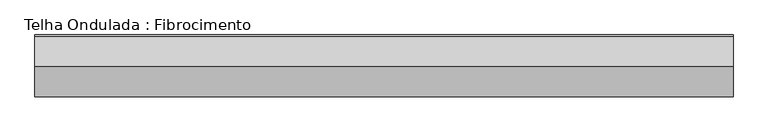
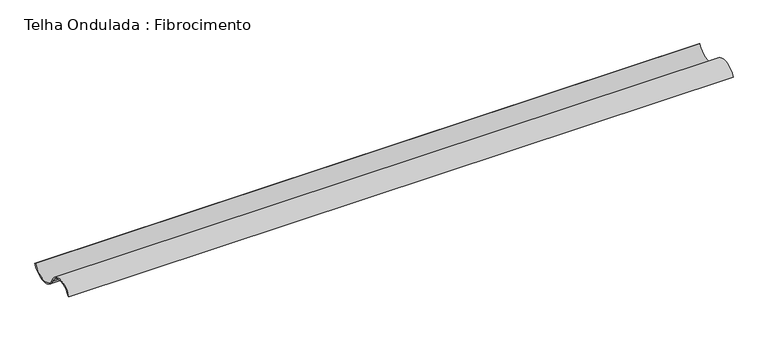
"""IFC4 building model written with IfcOpenShell, lengths in millimetres: beam geometry, Telha Ondulada : Fibrocimento."""

import ifcopenshell
import ifcopenshell.guid

model = None  # the IFC model being written
_history = None  # IfcOwnerHistory: only IFC2X3 demands one
_inside = {}  # id of a spatial element -> (the spatial element, [elements in it])
_under = {}  # id of a project, library or spatial element -> (it, [spatial elements below it])
_declared = {}  # id of a project -> (the project, [libraries it declares])
_typed = {}  # id of a type object -> (the type object, [elements of that type])
_made_of = {}  # id of a material, layer set ... -> (it, [elements and type objects made of it])


def new_model(schema):
    """Start an empty IFC model of exactly this schema.

    Asked for "IFC4X3", IfcOpenShell would pick the latest addendum, in which some entities
    have other attributes; the version numbers below select the first issue.
    IFC2X3 requires an IfcOwnerHistory on every rooted entity: one is made here for all.
    """
    global model, _history
    if schema == "IFC4X3":
        model = ifcopenshell.file(schema_version=(4, 3, 0, 0))
    else:
        model = ifcopenshell.file(schema=schema)
    _inside.clear()
    _under.clear()
    _declared.clear()
    _typed.clear()
    _made_of.clear()
    _history = None
    if model.schema == "IFC2X3":
        org = make("IfcOrganization", Name="unknown")
        user = make(
            "IfcPersonAndOrganization",
            ThePerson=make("IfcPerson", FamilyName="unknown"),
            TheOrganization=org,
        )
        app = make(
            "IfcApplication",
            ApplicationDeveloper=org,
            Version="unknown",
            ApplicationFullName="unknown",
            ApplicationIdentifier="unknown",
        )
        _history = make(
            "IfcOwnerHistory",
            OwningUser=user,
            OwningApplication=app,
            ChangeAction="ADDED",
            CreationDate=0,
        )
    return model


def make(cls, **values):
    """One entity of the class cls with the attributes given. An attribute that is None is left unset."""
    return model.create_entity(
        cls, **{name: value for name, value in values.items() if value is not None}
    )


def rooted(cls, **values):
    """An entity with a GlobalId (a new one), such as an element, a storey or a relation."""
    return make(cls, GlobalId=ifcopenshell.guid.new(), OwnerHistory=_history, **values)


def si_unit(unit_type, name, prefix=None):
    """IfcSIUnit, for example si_unit("LENGTHUNIT", "METRE", prefix="MILLI")."""
    return make("IfcSIUnit", UnitType=unit_type, Prefix=prefix, Name=name)


def assignment(units):
    """IfcUnitAssignment: the units of a project."""
    return None if units is None else make("IfcUnitAssignment", Units=units)


def point(xyz):
    """IfcCartesianPoint."""
    return None if xyz is None else make("IfcCartesianPoint", Coordinates=xyz)


def direction(xyz):
    """IfcDirection."""
    return None if xyz is None else make("IfcDirection", DirectionRatios=xyz)


def frame(location, z_axis=None, x_axis=None):
    """IfcAxis2Placement3D, a coordinate frame: its origin and axes. An axis left out is left unset."""
    return make(
        "IfcAxis2Placement3D",
        Location=point(location),
        Axis=direction(z_axis),
        RefDirection=direction(x_axis),
    )


def frame_2d(location, x_axis=None):
    """IfcAxis2Placement2D, a coordinate frame in the plane: its origin and x axis."""
    return make(
        "IfcAxis2Placement2D", Location=point(location), RefDirection=direction(x_axis)
    )


def origin():
    """The frame at (0, 0, 0) with its axes left unset."""
    return frame((0.0, 0.0, 0.0))


def place(relative_to, where):
    """IfcLocalPlacement: puts the frame where relative to a parent placement (None: the world)."""
    return make(
        "IfcLocalPlacement", PlacementRelTo=relative_to, RelativePlacement=where
    )


def context(
    kind, dimensions, precision=None, world=None, true_north=None, identifier=None
):
    """IfcGeometricRepresentationContext, for example the 3D "Model" context."""
    return make(
        "IfcGeometricRepresentationContext",
        ContextIdentifier=identifier,
        ContextType=kind,
        CoordinateSpaceDimension=dimensions,
        Precision=precision,
        WorldCoordinateSystem=world,
        TrueNorth=true_north,
    )


def project(units=None, contexts=None):
    """IfcProject with its units and contexts."""
    return rooted(
        "IfcProject",
        Name="project",
        RepresentationContexts=contexts,
        UnitsInContext=assignment(units),
    )


def spatial(cls, under=None, at=None, **own):
    """A site, building, storey or space (cls), placed at a placement, below another one or the project."""
    s = rooted(cls, ObjectPlacement=at, **own)
    if under is not None:
        _under.setdefault(under.id(), (under, []))[1].append(s)
    return s


def polyline(points):
    """IfcPolyline through the points."""
    return make("IfcPolyline", Points=[point(p) for p in points])


def circle_curve(where, radius):
    """IfcCircle in the frame where."""
    return make("IfcCircle", Position=where, Radius=radius)


def trimmed(basis, trim1, trim2, sense, master):
    """IfcTrimmedCurve: the piece of a basis curve between two trims."""
    return make(
        "IfcTrimmedCurve",
        BasisCurve=basis,
        Trim1=trim1,
        Trim2=trim2,
        SenseAgreement=sense,
        MasterRepresentation=master,
    )


def segment(curve, same_sense, transition):
    """IfcCompositeCurveSegment."""
    return make(
        "IfcCompositeCurveSegment",
        Transition=transition,
        SameSense=same_sense,
        ParentCurve=curve,
    )


def composite_curve(segments, self_intersect=None):
    """IfcCompositeCurve: segments joined end to end."""
    return make("IfcCompositeCurve", Segments=segments, SelfIntersect=self_intersect)


def outline(outer, holes=None, kind="AREA"):
    """IfcArbitraryClosedProfileDef: a profile drawn as a closed curve; with holes, ...WithVoids."""
    if holes is None:
        return make("IfcArbitraryClosedProfileDef", ProfileType=kind, OuterCurve=outer)
    return make(
        "IfcArbitraryProfileDefWithVoids",
        ProfileType=kind,
        OuterCurve=outer,
        InnerCurves=holes,
    )


def extrude(swept, where, along, depth):
    """IfcExtrudedAreaSolid: the profile swept, set in the frame where, extruded along a direction by depth."""
    return make(
        "IfcExtrudedAreaSolid",
        SweptArea=swept,
        Position=where,
        ExtrudedDirection=direction(along),
        Depth=depth,
    )


def shape(context_of_items, identifier, shape_type, items):
    """IfcShapeRepresentation: the items that make up one representation, for example the "Body"."""
    return make(
        "IfcShapeRepresentation",
        ContextOfItems=context_of_items,
        RepresentationIdentifier=identifier,
        RepresentationType=shape_type,
        Items=items,
    )


def source(mapping_origin, context_of_items, identifier, shape_type, items):
    """IfcRepresentationMap: a shape defined once, which mapped items show again and again."""
    return make(
        "IfcRepresentationMap",
        MappingOrigin=mapping_origin,
        MappedRepresentation=shape(context_of_items, identifier, shape_type, items),
    )


def transform(
    local_origin,
    x_axis=None,
    y_axis=None,
    z_axis=None,
    scale=None,
    scale2=None,
    scale3=None,
    uniform=True,
):
    """IfcCartesianTransformationOperator3D, or its non-uniform kind. x_axis, y_axis, z_axis: its Axis1, 2, 3."""
    if uniform:
        return make(
            "IfcCartesianTransformationOperator3D",
            Axis1=direction(x_axis),
            Axis2=direction(y_axis),
            LocalOrigin=point(local_origin),
            Scale=scale,
            Axis3=direction(z_axis),
        )
    return make(
        "IfcCartesianTransformationOperator3DnonUniform",
        Axis1=direction(x_axis),
        Axis2=direction(y_axis),
        LocalOrigin=point(local_origin),
        Scale=scale,
        Axis3=direction(z_axis),
        Scale2=scale2,
        Scale3=scale3,
    )


def mapped(mapping_source, mapping_target):
    """IfcMappedItem: shows the shape of a source again, moved by a transform."""
    return make(
        "IfcMappedItem", MappingSource=mapping_source, MappingTarget=mapping_target
    )


def made_of(thing, what):
    """Note that an element or type object is made of a material, layer set ...; save() writes the relation."""
    if what is not None:
        _made_of.setdefault(what.id(), (what, []))[1].append(thing)
    return thing


def element(
    cls,
    number,
    at=None,
    inside=None,
    cuts=None,
    type_object=None,
    material=None,
    context=None,
    identifier="Body",
    shape_type=None,
    held_by="IfcProductDefinitionShape",
    body=None,
    shapes=None,
    **own,
):
    """One element of the class cls, such as IfcWall. Its Tag is "e" and its number.

    at: its placement. inside: the storey or other place that contains it. cuts: it is an
    opening in that element (IfcRelVoidsElement). A single representation is given by context,
    identifier, shape_type and body (its items); several are given by shapes. held_by: the class
    of the entity that holds the representations. save() writes the other relations.
    """
    e = rooted(cls, Tag="e%d" % number, ObjectPlacement=at, **own)
    if body is not None:
        shapes = [shape(context, identifier, shape_type, body)]
    if shapes is not None:
        e.Representation = make(held_by, Representations=shapes)
    if inside is not None:
        _inside.setdefault(inside.id(), (inside, []))[1].append(e)
    if cuts is not None:
        rooted(
            "IfcRelVoidsElement", RelatingBuildingElement=cuts, RelatedOpeningElement=e
        )
    if type_object is not None:
        _typed.setdefault(type_object.id(), (type_object, []))[1].append(e)
    return made_of(e, material)


def aggregate(whole, parts):
    """IfcRelAggregates: a whole, such as a stair, and the parts it consists of."""
    return rooted("IfcRelAggregates", RelatingObject=whole, RelatedObjects=parts)


def save(model, path):
    """Write the relations noted so far, then the file.

    IfcRelAggregates (storeys below a building ...), IfcRelContainedInSpatialStructure (elements
    in a storey), IfcRelDefinesByType, IfcRelAssociatesMaterial and IfcRelDeclares: one each for
    every whole, place, type object, material and project.
    """
    for whole, parts in _under.values():
        aggregate(whole, parts)
    for where, things in _inside.values():
        rooted(
            "IfcRelContainedInSpatialStructure",
            RelatedElements=things,
            RelatingStructure=where,
        )
    for kind, things in _typed.values():
        rooted("IfcRelDefinesByType", RelatedObjects=things, RelatingType=kind)
    for what, things in _made_of.values():
        rooted("IfcRelAssociatesMaterial", RelatedObjects=things, RelatingMaterial=what)
    for by, libraries in _declared.values():
        rooted("IfcRelDeclares", RelatingContext=by, RelatedDefinitions=libraries)
    model.write(path)


def telha_ondulada_fibrocimento_bfc377d9(model_context):
    return source(origin(), model_context, "Body", "SweptSolid", [
        extrude(outline(composite_curve([segment(trimmed(circle_curve(frame_2d((68.3970135, 71.7939461)), 66.7939461), [point((8.3970135, 42.4437972))], [point((128.3970135, 42.4437972))], True, "CARTESIAN"), True, "CONTINUOUS"), segment(polyline([(128.3970135, 42.4437972), (132.8884385, 40.2467307)]), True, "CONTINUOUS"), segment(trimmed(circle_curve(frame_2d((68.3970135, 71.7939461)), 71.7939461), [point((132.8884385, 40.2467307))], [point((3.9055884, 40.2467307))], False, "CARTESIAN"), True, "CONTINUOUS"), segment(trimmed(circle_curve(frame_2d((-51.6029865, 13.0936483)), 61.7939461), [point((3.9055884, 40.2467307))], [point((-107.1115615, 40.2467307))], True, "CARTESIAN"), True, "CONTINUOUS"), segment(polyline([(-107.1115615, 40.2467307), (-111.6029865, 42.4437972)]), True, "CONTINUOUS"), segment(trimmed(circle_curve(frame_2d((-51.6029865, 13.0936483)), 66.7939461), [point((-111.6029865, 42.4437972))], [point((8.3970135, 42.4437972))], False, "CARTESIAN"), True, "CONTINUOUS")], self_intersect=False)), frame((-1382.2210865, 0.0, 0.0), z_axis=(1.0, 0.0, 0.0), x_axis=(0.0, 1.0, 0.0)), (0.0, 0.0, 1.0), 2764.442173),
    ])


if __name__ == "__main__":
    model = new_model("IFC4")
    model_context = context("Model", 3, world=origin())
    ifc_project = project(units=[si_unit("LENGTHUNIT", "METRE", prefix="MILLI")], contexts=[model_context])
    site = spatial("IfcSite", under=ifc_project)
    building = spatial("IfcBuilding", under=site)
    placement = place(None, origin())
    telha_ondulada_fibrocimento_shape = telha_ondulada_fibrocimento_bfc377d9(model_context)
    element("IfcBeam", 1, ObjectType="Telha Ondulada : Fibrocimento", at=placement, inside=building, context=model_context, shape_type="MappedRepresentation", body=[
        mapped(telha_ondulada_fibrocimento_shape, transform((0.0, 0.0, 0.0), x_axis=(1.0, 0.0, 0.0), y_axis=(0.0, 1.0, 0.0), z_axis=(0.0, 0.0, 1.0))),
    ])
    save(model, "model.ifc")

# Revit data of these elements
# Type "Telha Ondulada : Fibrocimento"
#   Description = "TELHA ONDULADA FIBROCIMENTO"
#   Cost = 5
#   Length [instance default] = 1.524 m
#   b = 0.07 m
#   h = 0.16 m
#   Structural Material = .TELHA DE FIBROCIMENTO
#   Assembly Code = ""
# Element 1 (IfcBeam, "Telha Ondulada : Fibrocimento")
#   Materials on its faces: ".TELHA DE FIBROCIMENTO"
# Materials
#   ".TELHA DE FIBROCIMENTO": class "CC_TELHADO", colour RGB 77 77 76, transparency 0, Description = "TELHA ONDULADA FIBROCIMENTO", Cost = 0
